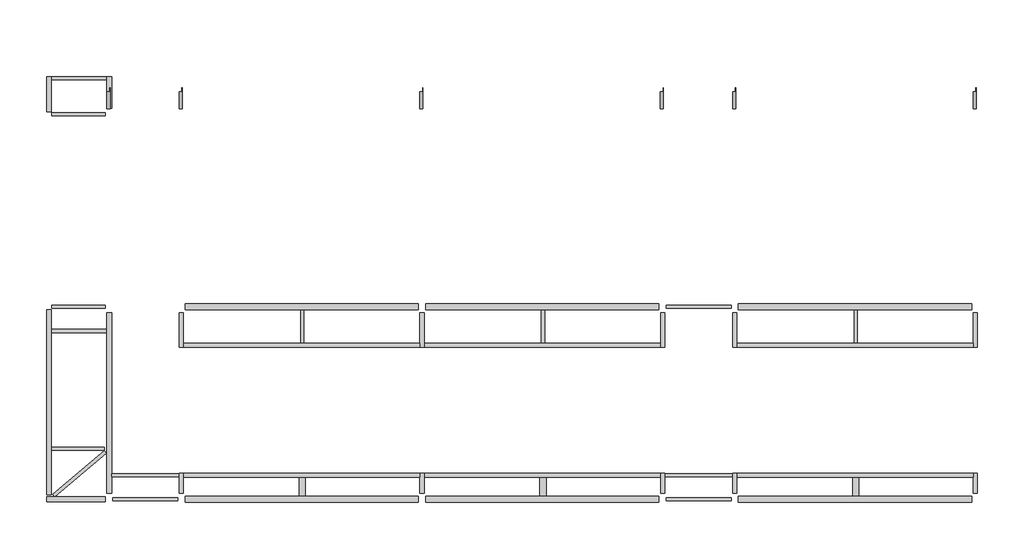
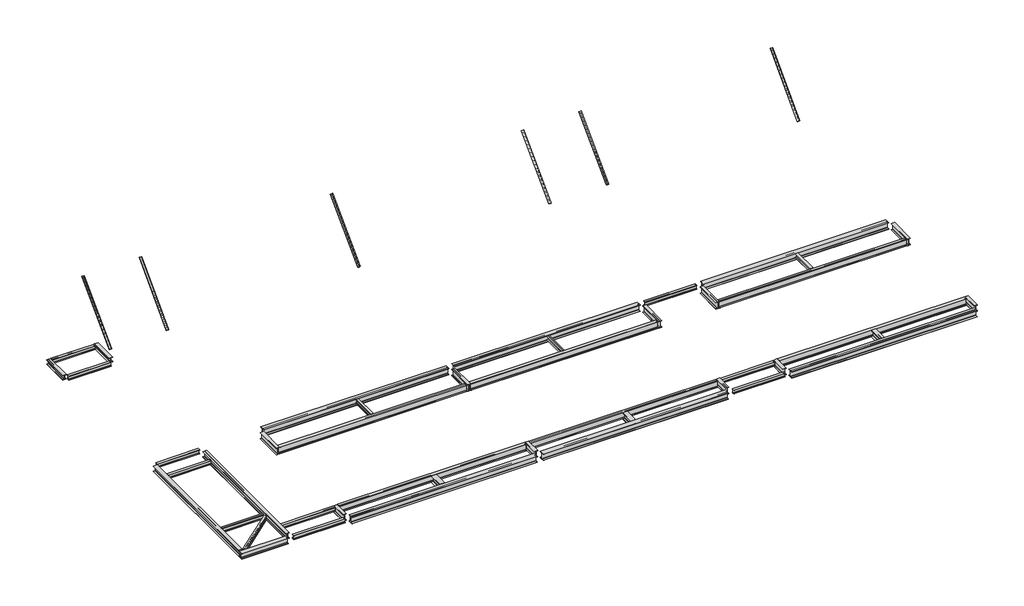
# One storey: 44 beams, 6 members.
# Revit data of these elements (continued)
# Project information (continued)
#   Project Address = "서울시 종로구 율곡로 75(계동)"
#   Project Number = "-"
# Grids (mm)
#   "D": line (-6469.284, 22499.521) -> (39003.298, 22499.521)
#   "1": line (0, 24502.793) -> (0, -3987.031)
#   "3": line (13000, 24502.793) -> (13000, -3987.031)
#   "B": line (-6469.284, 6499.521) -> (39003.298, 6499.521)
#   "A": line (-6469.284, 499.521) -> (39003.298, 499.521)
#   "4": line (23000, 24502.793) -> (23000, -3987.031)
#   "5": line (26000, 24502.793) -> (26000, -3987.031)
#   "6": line (36000, 24502.793) -> (36000, -3987.031)
#   "1 A": line (-2500, 24502.793) -> (-2500, 12276.643)
#   "2": line (3000, 24502.793) -> (3000, -3987.031)
#   "7": line (1307.038, 15699.521) -> (-4718.233, 15699.521)
#   "8": line (1307.038, 17449.521) -> (-4718.233, 17449.521)
#   "9": line (5528.605, 13006.092) -> (5528.605, 16811.527)
#   "10": line (8028.605, 13006.092) -> (8028.605, 16811.527)
#   "11": line (10528.605, 13006.092) -> (10528.605, 16811.527)
#   "12": line (20528.605, 13006.092) -> (20528.605, 16811.527)
#   "13": line (18028.605, 13006.092) -> (18028.605, 16811.527)
#   "14": line (15528.605, 13006.092) -> (15528.605, 16811.527)
#   "15": line (18000, -1079.942) -> (18000, 22499.521)
#   "16": line (27211.823, 9169.521) -> (22203.608, 9169.521)
#   "17": line (3430.624, 9199.521) -> (-461.103, 9199.521)
#   "18": line (4961.493, 9299.521) -> (2471.526, 9299.521)
#   "19": line (20500, 22120.772) -> (20500, 25499.521)
#   "20": line (15500, 22120.772) -> (15500, 25499.521)
#   "21": line (10500, 22120.772) -> (10500, 25499.521)
#   "22": line (5500, 22120.772) -> (5500, 25499.521)
#   "23": line (-6469.284, -2000.479) -> (39003.298, -2000.479)
#   "C": line (-6469.284, 14499.521) -> (39003.298, 14499.521)
# Type "Steel Framing_W_ASTM A6M : H_SB_AR_S02_W200x31.3_B6"
#   Type Mark = "B6"
#   Section Name Key = "W8x21"
#   Width = 13.4 cm
#   Web Thickness = 0.635 cm
#   Web Fillet = 0.76 cm
#   Warping Constant = 40800.0 cm⁶
#   Torsional Moment of Inertia = 11.70 cm⁴
#   Section Area = 39.7 cm²
#   Plastic Modulus weak axis = 93.2 cm³
#   Plastic Modulus strong axis = 334.0 cm³
#   Perimeter = 0.93 m²/m
#   Nominal Weight = 31.30 kgf/m
#   Moment of Inertia weak axis = 407.00 cm⁴
#   Moment of Inertia strong axis = 3130.00 cm⁴
#   Height = 21.0 cm
#   Flange Thickness = 1.02 cm
#   Elastic Modulus weak axis = 60.8 cm³
#   Elastic Modulus strong axis = 298.0 cm³
#   Centroid Vertical = 10.5 cm
#   Centroid Horizontal = 6.7 cm
#   Length [instance default] = 1500 mm
#   Structural Material [instance default] = Steel, 45-345
#   Bolt Spacing = 0
#   Assembly Code = ""
# Type "Steel Framing_W_ASTM A6M : H_SB_AR_S02_W360x91_B3"
#   Type Mark = "B3"
#   Section Name Key = "W14x61"
#   Width = 25.4 cm
#   Web Thickness = 0.953 cm
#   Web Fillet = 1.51 cm
#   Warping Constant = 1260000.0 cm⁶
#   Torsional Moment of Inertia = 91.20 cm⁴
#   Section Area = 115.0 cm²
#   Plastic Modulus weak axis = 537.0 cm³
#   Plastic Modulus strong axis = 1670.0 cm³
#   Perimeter = 1.68 m²/m
#   Nominal Weight = 91.00 kgf/m
#   Moment of Inertia weak axis = 4450.00 cm⁴
#   Moment of Inertia strong axis = 26600.00 cm⁴
#   Height = 35.3 cm
#   Flange Thickness = 1.64 cm
#   Elastic Modulus weak axis = 352.0 cm³
#   Elastic Modulus strong axis = 1510.0 cm³
#   Centroid Vertical = 17.65 cm
#   Centroid Horizontal = 12.7 cm
#   Length [instance default] = 1500 mm
#   Structural Material [instance default] = Steel, 45-345
#   Bolt Spacing = 0
#   Assembly Code = ""
# Type "Steel Framing_W_ASTM A6M : H_SB_AR_S02_W310x60_G4"
#   Type Mark = "G4"
#   Section Name Key = "W12x40"
#   Width = 20.3 cm
#   Web Thickness = 0.749 cm
#   Web Fillet = 1.28 cm
#   Warping Constant = 387000.0 cm⁶
#   Torsional Moment of Inertia = 37.70 cm⁴
#   Section Area = 75.5 cm²
#   Plastic Modulus weak axis = 275.0 cm³
#   Plastic Modulus strong axis = 934.0 cm³
#   Perimeter = 1.38 m²/m
#   Nominal Weight = 60.00 kgf/m
#   Moment of Inertia weak axis = 1840.00 cm⁴
#   Moment of Inertia strong axis = 12800.00 cm⁴
#   Height = 30.2 cm
#   Flange Thickness = 1.31 cm
#   Elastic Modulus weak axis = 180.0 cm³
#   Elastic Modulus strong axis = 844.0 cm³
#   Centroid Vertical = 15.1 cm
#   Centroid Horizontal = 10.15 cm
#   Length [instance default] = 1500 mm
#   Structural Material [instance default] = Steel, 45-345
#   Bolt Spacing = 0
#   Assembly Code = ""
# Type "Steel Framing_W_ASTM A6M : H_SB_AR_S02_W250x49.1_G5"
#   Type Mark = "G5"
#   Section Name Key = "W10x33"
#   Width = 20.2 cm
#   Web Thickness = 0.737 cm
#   Web Fillet = 1.27 cm
#   Warping Constant = 212000.0 cm⁶
#   Torsional Moment of Inertia = 24.30 cm⁴
#   Section Area = 62.6 cm²
#   Plastic Modulus weak axis = 229.0 cm³
#   Plastic Modulus strong axis = 636.0 cm³
#   Perimeter = 1.27 m²/m
#   Nominal Weight = 49.10 kgf/m
#   Moment of Inertia weak axis = 1520.00 cm⁴
#   Moment of Inertia strong axis = 7120.00 cm⁴
#   Height = 24.7 cm
#   Flange Thickness = 1.1 cm
#   Elastic Modulus weak axis = 151.0 cm³
#   Elastic Modulus strong axis = 574.0 cm³
#   Centroid Vertical = 12.35 cm
#   Centroid Horizontal = 10.1 cm
#   Length [instance default] = 1500 mm
#   Structural Material [instance default] = Steel, 45-345
#   Bolt Spacing = 0
#   Assembly Code = ""
# Type "Steel Framing_W_ASTM A6M : H_SB_AR_S02_W310x60_B5"
#   Type Mark = "B5"
#   Section Name Key = "W12x40"
#   Width = 20.3 cm
#   Web Thickness = 0.749 cm
#   Web Fillet = 1.28 cm
#   Warping Constant = 387000.0 cm⁶
#   Torsional Moment of Inertia = 37.70 cm⁴
#   Section Area = 75.5 cm²
#   Plastic Modulus weak axis = 275.0 cm³
#   Plastic Modulus strong axis = 934.0 cm³
#   Perimeter = 1.38 m²/m
#   Nominal Weight = 60.00 kgf/m
#   Moment of Inertia weak axis = 1840.00 cm⁴
#   Moment of Inertia strong axis = 12800.00 cm⁴
#   Height = 30.2 cm
#   Flange Thickness = 1.31 cm
#   Elastic Modulus weak axis = 180.0 cm³
#   Elastic Modulus strong axis = 844.0 cm³
#   Centroid Vertical = 15.1 cm
#   Centroid Horizontal = 10.15 cm
#   Length [instance default] = 1500 mm
#   Structural Material [instance default] = Steel, 45-345
#   Bolt Spacing = 0
#   Assembly Code = ""
# Type "Steel Framing_W_ASTM A6M : H_SB_AR_S02_W360x51_G3"
#   Type Mark = "G3"
#   Section Name Key = "W14x34"
#   Width = 17.1 cm
#   Web Thickness = 0.724 cm
#   Web Fillet = 1.01 cm
#   Warping Constant = 287000.0 cm⁶
#   Torsional Moment of Inertia = 23.70 cm⁴
#   Section Area = 64.5 cm²
#   Plastic Modulus weak axis = 174.0 cm³
#   Plastic Modulus strong axis = 895.0 cm³
#   Perimeter = 1.36 m²/m
#   Nominal Weight = 51.00 kgf/m
#   Moment of Inertia weak axis = 970.00 cm⁴
#   Moment of Inertia strong axis = 14200.00 cm⁴
#   Height = 35.6 cm
#   Flange Thickness = 1.16 cm
#   Elastic Modulus weak axis = 113.0 cm³
#   Elastic Modulus strong axis = 796.0 cm³
#   Centroid Vertical = 17.8 cm
#   Centroid Horizontal = 8.55 cm
#   Length [instance default] = 1500 mm
#   Structural Material [instance default] = Steel, 45-345
#   Bolt Spacing = 0
#   Assembly Code = ""
# Type "Steel Framing_W_ASTM A6M : H_SB_AR_S02_W360x51_B4"
#   Type Mark = "B4"
#   Section Name Key = "W14x34"
#   Width = 17.1 cm
#   Web Thickness = 0.724 cm
#   Web Fillet = 1.01 cm
#   Warping Constant = 287000.0 cm⁶
#   Torsional Moment of Inertia = 23.70 cm⁴
#   Section Area = 64.5 cm²
#   Plastic Modulus weak axis = 174.0 cm³
#   Plastic Modulus strong axis = 895.0 cm³
#   Perimeter = 1.36 m²/m
#   Nominal Weight = 51.00 kgf/m
#   Moment of Inertia weak axis = 970.00 cm⁴
#   Moment of Inertia strong axis = 14200.00 cm⁴
#   Height = 35.6 cm
#   Flange Thickness = 1.16 cm
#   Elastic Modulus weak axis = 113.0 cm³
#   Elastic Modulus strong axis = 796.0 cm³
#   Centroid Vertical = 17.8 cm
#   Centroid Horizontal = 8.55 cm
#   Length [instance default] = 1500 mm
#   Structural Material [instance default] = Steel, 45-345
#   Bolt Spacing = 0
#   Assembly Code = ""
# Type "0912_Steel Framing_L-KSD3502 : H_SB_AR_S04_L-130x130x12_KBR1"
#   k = 25 mm
#   Perimeter = 0.52 m²/m
#   Nominal Weight = 23.40 kgf/m
#   Length [instance default] = 1000 mm
#   b = 130 mm
#   d = 130 mm
#   t = 12 mm
#   x = 36.4 mm
#   y = 36.4 mm
#   A = 2976.00 m²
#   Structural Material [instance default] = Steel, 45-345
# Elements 1, 2, 3, 4, 5, 6, 15, 17, 19, 21, 22, 39, 40, 41 (IfcBeam, "Steel Framing_W_ASTM A6M : H_SB_AR_S02_W200x31.3_B6")
#   Structural Material = Steel, 45-345
#   Phase Created = New Construction
#   Materials on its faces: "Steel, 45-345"
# Elements 7, 8, 9, 10, 11, 12, 42, 43, 44 (IfcBeam, "Steel Framing_W_ASTM A6M : H_SB_AR_S02_W360x91_B3")
#   Structural Material = Steel, 45-345
#   Phase Created = New Construction
#   Materials on its faces: "Steel, 45-345"
# Element 13 (IfcBeam, "Steel Framing_W_ASTM A6M : H_SB_AR_S02_W310x60_G4")
#   Structural Material = Steel, 45-345
#   Phase Created = New Construction
#   Materials on its faces: "Steel, 45-345"
# Elements 14, 16 (IfcBeam, "Steel Framing_W_ASTM A6M : H_SB_AR_S02_W250x49.1_G5")
#   Length = 1500 mm
#   Structural Material = Steel, 45-345
#   Phase Created = New Construction
#   Materials on its faces: "Steel, 45-345"
# Elements 18, 20 (IfcBeam, "Steel Framing_W_ASTM A6M : H_SB_AR_S02_W310x60_B5")
#   Structural Material = Steel, 45-345
#   Phase Created = New Construction
#   Materials on its faces: "Steel, 45-345"
# Elements 23, 24, 25, 26, 27, 34, 35, 36, 37, 38 (IfcBeam, "Steel Framing_W_ASTM A6M : H_SB_AR_S02_W360x51_G3")
#   Structural Material = Steel, 45-345
#   Phase Created = New Construction
#   Materials on its faces: "Steel, 45-345"
# Elements 28, 29, 30, 31, 32, 33 (IfcBeam, "Steel Framing_W_ASTM A6M : H_SB_AR_S02_W360x51_B4")
#   Structural Material = Steel, 45-345
#   Phase Created = New Construction
#   Materials on its faces: "Steel, 45-345"
# Elements 45, 46, 47, 48, 49, 50 (IfcMember, "0912_Steel Framing_L-KSD3502 : H_SB_AR_S04_L-130x130x12_KBR1")
#   Structural Material = Steel, 45-345
#   Phase Created = New Construction
#   Materials on its faces: "Steel, 45-345"
# Materials
#   "Steel, 45-345": class "Metal", colour RGB 189 187 185, transparency 0, Description = "Steel 345 MPa", Cost = 0
